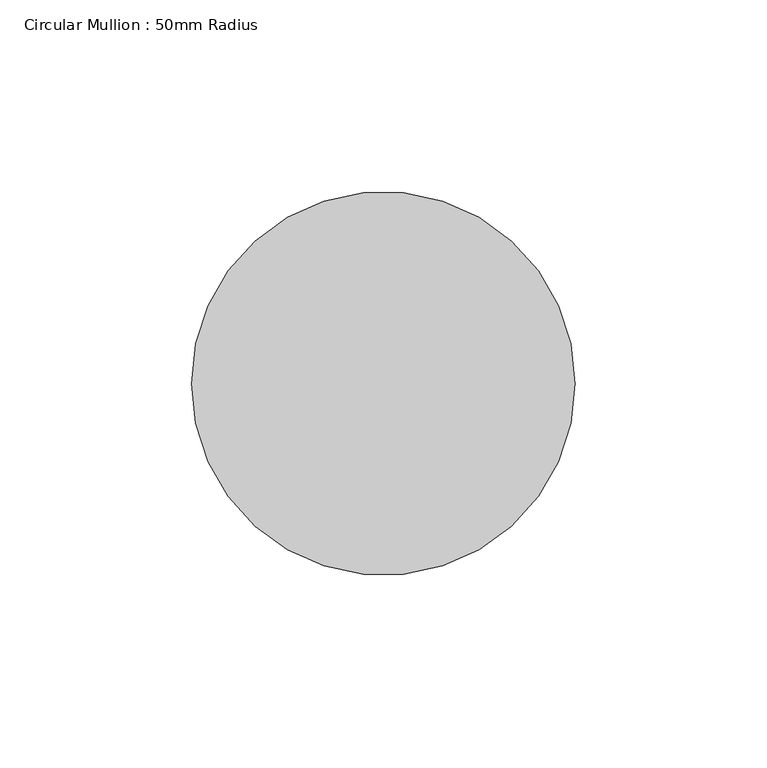
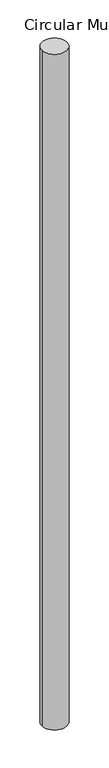
"""IFC4 building model written with IfcOpenShell, lengths in millimetres: member geometry, Circular Mullion : 50mm Radius."""

from ifc_helpers import new_model, si_unit, point, frame, frame_2d, origin, place, context, project, spatial, circle_curve, trimmed, segment, composite_curve, outline, extrude, source, transform, mapped, element, save


def circular_mullion_50mm_radius_4545dc5f(model_context):
    return source(origin(), model_context, "Body", "SweptSolid", [
        extrude(outline(composite_curve([segment(trimmed(circle_curve(frame_2d((-50.0, 0.0)), 50.0), [point((0.0, 0.0))], [point((-100.0, 0.0))], False, "CARTESIAN"), True, "CONTINUOUS"), segment(trimmed(circle_curve(frame_2d((-50.0, 0.0)), 50.0), [point((-100.0, 0.0))], [point((0.0, 0.0))], False, "CARTESIAN"), True, "CONTINUOUS")], self_intersect=False)), frame((0.0, 0.0, -2854.1930266), z_axis=(0.0, 0.0, 1.0), x_axis=(1.0, 0.0, 0.0)), (0.0, 0.0, 1.0), 2854.1930266),
    ])


if __name__ == "__main__":
    model = new_model("IFC4")
    model_context = context("Model", 3, world=origin())
    ifc_project = project(units=[si_unit("LENGTHUNIT", "METRE", prefix="MILLI")], contexts=[model_context])
    site = spatial("IfcSite", under=ifc_project)
    building = spatial("IfcBuilding", under=site)
    placement = place(None, origin())
    circular_mullion_50mm_radius_shape = circular_mullion_50mm_radius_4545dc5f(model_context)
    element("IfcMember", 1, ObjectType="Circular Mullion : 50mm Radius", at=placement, inside=building, context=model_context, shape_type="MappedRepresentation", body=[
        mapped(circular_mullion_50mm_radius_shape, transform((0.0, 0.0, 0.0), x_axis=(1.0, 0.0, 0.0), y_axis=(0.0, 1.0, 0.0), z_axis=(0.0, 0.0, 1.0))),
    ])
    save(model, "model.ifc")

# Revit data of these elements
# Type "Circular Mullion : 50mm Radius"
#   built-in parameter 1007350 = 0.164042 (stored number, unit not read)
# Element 1 (IfcMember, "Circular Mullion : 50mm Radius")
#   Materials on its faces: "Aluminium"
# Materials
#   "Aluminium": class "Metal", colour RGB 247 247 247, transparency 0, Description = "Aluminium 6061", Cost = 0
